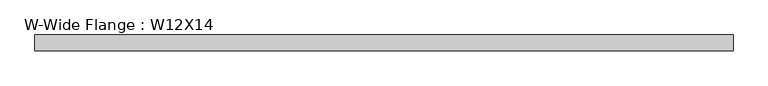
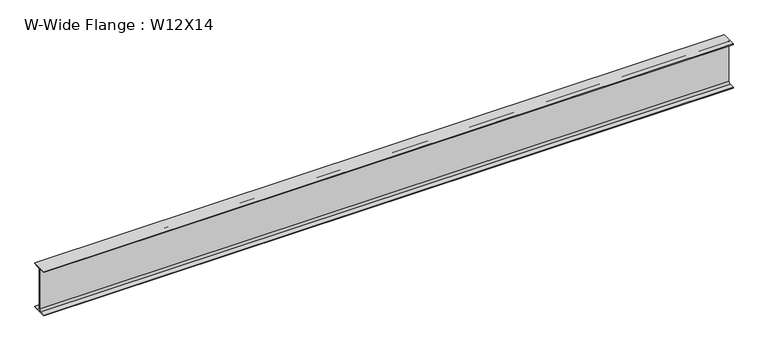
"""IFC4 building model written with IfcOpenShell, lengths in millimetres: beam geometry, W-Wide Flange : W12X14."""

from ifc_helpers import new_model, si_unit, point, frame, frame_2d, origin, place, context, project, spatial, polyline, circle_curve, trimmed, segment, composite_curve, outline, extrude, source, transform, mapped, element, save


def w_wide_flange_w12x14_ab30ef1d(model_context):
    return source(origin(), model_context, "Body", "SweptSolid", [
        extrude(outline(composite_curve([segment(polyline([(50.419, -145.415), (50.419, -151.13), (-50.419, -151.13), (-50.419, -145.415), (-15.875, -145.415)]), True, "CONTINUOUS"), segment(trimmed(circle_curve(frame_2d((-15.875, -132.08)), 13.335), [point((-15.875, -145.415))], [point((-2.54, -132.08))], True, "CARTESIAN"), True, "CONTINUOUS"), segment(polyline([(-2.54, -132.08), (-2.54, 132.08)]), True, "CONTINUOUS"), segment(trimmed(circle_curve(frame_2d((-15.875, 132.08)), 13.335), [point((-2.54, 132.08))], [point((-15.875, 145.415))], True, "CARTESIAN"), True, "CONTINUOUS"), segment(polyline([(-15.875, 145.415), (-50.419, 145.415), (-50.419, 151.13), (50.419, 151.13), (50.419, 145.415), (15.875, 145.415)]), True, "CONTINUOUS"), segment(trimmed(circle_curve(frame_2d((15.875, 132.08)), 13.335), [point((15.875, 145.415))], [point((2.54, 132.08))], True, "CARTESIAN"), True, "CONTINUOUS"), segment(polyline([(2.54, 132.08), (2.54, -132.08)]), True, "CONTINUOUS"), segment(trimmed(circle_curve(frame_2d((15.875, -132.08)), 13.335), [point((2.54, -132.08))], [point((15.875, -145.415))], True, "CARTESIAN"), True, "CONTINUOUS"), segment(polyline([(15.875, -145.415), (50.419, -145.415)]), True, "CONTINUOUS")], self_intersect=False)), frame((-2235.2, 0.0, 0.0), z_axis=(1.0, 0.0, 0.0), x_axis=(0.0, 1.0, 0.0)), (0.0, 0.0, 1.0), 4451.35),
    ])


if __name__ == "__main__":
    model = new_model("IFC4")
    model_context = context("Model", 3, world=origin())
    ifc_project = project(units=[si_unit("LENGTHUNIT", "METRE", prefix="MILLI")], contexts=[model_context])
    site = spatial("IfcSite", under=ifc_project)
    building = spatial("IfcBuilding", under=site)
    placement = place(None, origin())
    w_wide_flange_w12x14_shape = w_wide_flange_w12x14_ab30ef1d(model_context)
    element("IfcBeam", 1, ObjectType="W-Wide Flange : W12X14", at=placement, inside=building, context=model_context, shape_type="MappedRepresentation", body=[
        mapped(w_wide_flange_w12x14_shape, transform((0.0, 0.0, 0.0), x_axis=(1.0, 0.0, 0.0), y_axis=(0.0, 1.0, 0.0), z_axis=(0.0, 0.0, 1.0))),
    ])
    save(model, "model.ifc")

# Revit data of these elements
# Type "W-Wide Flange : W12X14"
#   Assembly Code = "B10"
#   W = 14
#   Length [instance default] = 5' - 0"
#   bf = 0' - 3.97"
#   d = 0' - 11.9"
#   k = 0' - 0 3/4"
#   k2 = 0' - 0.525"
#   tf = 0' - 0.225"
#   tw = 0' - 0.2"
#   A = 0.0288889 SF
#   Structural Material [instance default] = Steel ASTM A992
# Element 1 (IfcBeam, "W-Wide Flange : W12X14")
#   Materials on its faces: "Steel ASTM A992"
# Materials
#   "Steel ASTM A992": class "Metal", colour RGB 199 199 199, transparency 0, Description = "Structural steel 50ksi", Cost = 0
